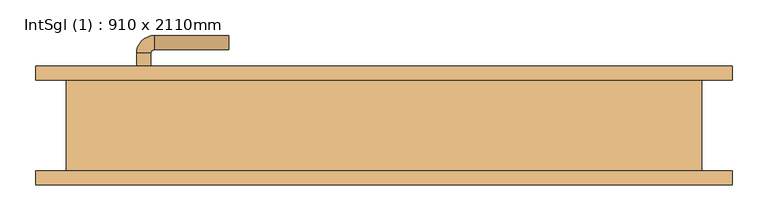
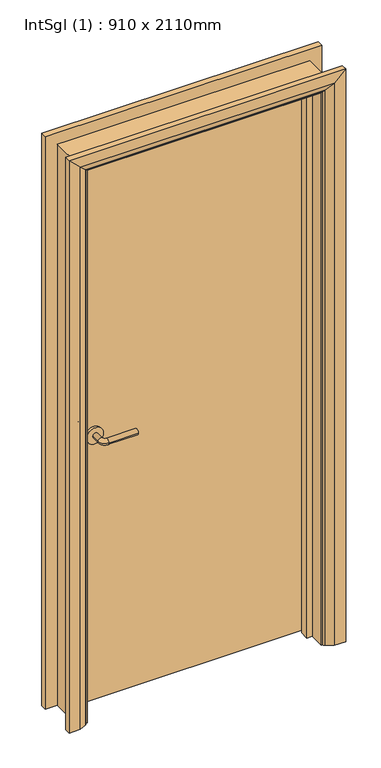
"""IFC4 building model written with IfcOpenShell, lengths in millimetres: door geometry, IntSgl (1) : 910 x 2110mm."""

import ifcopenshell
import ifcopenshell.guid

model = None  # the IFC model being written
_history = None  # IfcOwnerHistory: only IFC2X3 demands one
_inside = {}  # id of a spatial element -> (the spatial element, [elements in it])
_under = {}  # id of a project, library or spatial element -> (it, [spatial elements below it])
_declared = {}  # id of a project -> (the project, [libraries it declares])
_typed = {}  # id of a type object -> (the type object, [elements of that type])
_made_of = {}  # id of a material, layer set ... -> (it, [elements and type objects made of it])


def new_model(schema):
    """Start an empty IFC model of exactly this schema.

    Asked for "IFC4X3", IfcOpenShell would pick the latest addendum, in which some entities
    have other attributes; the version numbers below select the first issue.
    IFC2X3 requires an IfcOwnerHistory on every rooted entity: one is made here for all.
    """
    global model, _history
    if schema == "IFC4X3":
        model = ifcopenshell.file(schema_version=(4, 3, 0, 0))
    else:
        model = ifcopenshell.file(schema=schema)
    _inside.clear()
    _under.clear()
    _declared.clear()
    _typed.clear()
    _made_of.clear()
    _history = None
    if model.schema == "IFC2X3":
        org = make("IfcOrganization", Name="unknown")
        user = make(
            "IfcPersonAndOrganization",
            ThePerson=make("IfcPerson", FamilyName="unknown"),
            TheOrganization=org,
        )
        app = make(
            "IfcApplication",
            ApplicationDeveloper=org,
            Version="unknown",
            ApplicationFullName="unknown",
            ApplicationIdentifier="unknown",
        )
        _history = make(
            "IfcOwnerHistory",
            OwningUser=user,
            OwningApplication=app,
            ChangeAction="ADDED",
            CreationDate=0,
        )
    return model


def make(cls, **values):
    """One entity of the class cls with the attributes given. An attribute that is None is left unset."""
    return model.create_entity(
        cls, **{name: value for name, value in values.items() if value is not None}
    )


def rooted(cls, **values):
    """An entity with a GlobalId (a new one), such as an element, a storey or a relation."""
    return make(cls, GlobalId=ifcopenshell.guid.new(), OwnerHistory=_history, **values)


def si_unit(unit_type, name, prefix=None):
    """IfcSIUnit, for example si_unit("LENGTHUNIT", "METRE", prefix="MILLI")."""
    return make("IfcSIUnit", UnitType=unit_type, Prefix=prefix, Name=name)


def assignment(units):
    """IfcUnitAssignment: the units of a project."""
    return None if units is None else make("IfcUnitAssignment", Units=units)


def point(xyz):
    """IfcCartesianPoint."""
    return None if xyz is None else make("IfcCartesianPoint", Coordinates=xyz)


def direction(xyz):
    """IfcDirection."""
    return None if xyz is None else make("IfcDirection", DirectionRatios=xyz)


def frame(location, z_axis=None, x_axis=None):
    """IfcAxis2Placement3D, a coordinate frame: its origin and axes. An axis left out is left unset."""
    return make(
        "IfcAxis2Placement3D",
        Location=point(location),
        Axis=direction(z_axis),
        RefDirection=direction(x_axis),
    )


def frame_2d(location, x_axis=None):
    """IfcAxis2Placement2D, a coordinate frame in the plane: its origin and x axis."""
    return make(
        "IfcAxis2Placement2D", Location=point(location), RefDirection=direction(x_axis)
    )


def origin():
    """The frame at (0, 0, 0) with its axes left unset."""
    return frame((0.0, 0.0, 0.0))


def place(relative_to, where):
    """IfcLocalPlacement: puts the frame where relative to a parent placement (None: the world)."""
    return make(
        "IfcLocalPlacement", PlacementRelTo=relative_to, RelativePlacement=where
    )


def context(
    kind, dimensions, precision=None, world=None, true_north=None, identifier=None
):
    """IfcGeometricRepresentationContext, for example the 3D "Model" context."""
    return make(
        "IfcGeometricRepresentationContext",
        ContextIdentifier=identifier,
        ContextType=kind,
        CoordinateSpaceDimension=dimensions,
        Precision=precision,
        WorldCoordinateSystem=world,
        TrueNorth=true_north,
    )


def project(units=None, contexts=None):
    """IfcProject with its units and contexts."""
    return rooted(
        "IfcProject",
        Name="project",
        RepresentationContexts=contexts,
        UnitsInContext=assignment(units),
    )


def spatial(cls, under=None, at=None, **own):
    """A site, building, storey or space (cls), placed at a placement, below another one or the project."""
    s = rooted(cls, ObjectPlacement=at, **own)
    if under is not None:
        _under.setdefault(under.id(), (under, []))[1].append(s)
    return s


def polyline(points):
    """IfcPolyline through the points."""
    return make("IfcPolyline", Points=[point(p) for p in points])


def circle_curve(where, radius):
    """IfcCircle in the frame where."""
    return make("IfcCircle", Position=where, Radius=radius)


def ellipse_curve(where, semi_axis1, semi_axis2):
    """IfcEllipse in the frame where."""
    return make(
        "IfcEllipse", Position=where, SemiAxis1=semi_axis1, SemiAxis2=semi_axis2
    )


def trimmed(basis, trim1, trim2, sense, master):
    """IfcTrimmedCurve: the piece of a basis curve between two trims."""
    return make(
        "IfcTrimmedCurve",
        BasisCurve=basis,
        Trim1=trim1,
        Trim2=trim2,
        SenseAgreement=sense,
        MasterRepresentation=master,
    )


def segment(curve, same_sense, transition):
    """IfcCompositeCurveSegment."""
    return make(
        "IfcCompositeCurveSegment",
        Transition=transition,
        SameSense=same_sense,
        ParentCurve=curve,
    )


def composite_curve(segments, self_intersect=None):
    """IfcCompositeCurve: segments joined end to end."""
    return make("IfcCompositeCurve", Segments=segments, SelfIntersect=self_intersect)


def outline(outer, holes=None, kind="AREA"):
    """IfcArbitraryClosedProfileDef: a profile drawn as a closed curve; with holes, ...WithVoids."""
    if holes is None:
        return make("IfcArbitraryClosedProfileDef", ProfileType=kind, OuterCurve=outer)
    return make(
        "IfcArbitraryProfileDefWithVoids",
        ProfileType=kind,
        OuterCurve=outer,
        InnerCurves=holes,
    )


def extrude(swept, where, along, depth):
    """IfcExtrudedAreaSolid: the profile swept, set in the frame where, extruded along a direction by depth."""
    return make(
        "IfcExtrudedAreaSolid",
        SweptArea=swept,
        Position=where,
        ExtrudedDirection=direction(along),
        Depth=depth,
    )


def faces_of(points, faces, orient=None, outer=None):
    """IfcFace entities. A face is a list of loops; a loop is a list of indices into points, from 0.

    orient and outer hold one flag for each loop. By default every Orientation is true, the
    first loop of a face is its IfcFaceOuterBound and the others are IfcFaceBound.
    """
    made = []
    for i, loops in enumerate(faces):
        bounds = []
        for j, loop in enumerate(loops):
            is_outer = j == 0 if outer is None else outer[i][j]
            bounds.append(
                make(
                    "IfcFaceOuterBound" if is_outer else "IfcFaceBound",
                    Bound=make("IfcPolyLoop", Polygon=[points[k] for k in loop]),
                    Orientation=True if orient is None else orient[i][j],
                )
            )
        made.append(make("IfcFace", Bounds=bounds))
    return made


def faceted_brep(points, faces, orient=None, outer=None, voids=None):
    """IfcFacetedBrep: a solid bounded by flat faces; with voids (closed shells), ...WithVoids."""
    shared = [point(p) for p in points]
    hull = make("IfcClosedShell", CfsFaces=faces_of(shared, faces, orient, outer))
    if voids is None:
        return make("IfcFacetedBrep", Outer=hull)
    return make(
        "IfcFacetedBrepWithVoids",
        Outer=hull,
        Voids=[
            make(cls, CfsFaces=faces_of(shared, fs, o, b)) for cls, fs, o, b in voids
        ],
    )


def shape(context_of_items, identifier, shape_type, items):
    """IfcShapeRepresentation: the items that make up one representation, for example the "Body"."""
    return make(
        "IfcShapeRepresentation",
        ContextOfItems=context_of_items,
        RepresentationIdentifier=identifier,
        RepresentationType=shape_type,
        Items=items,
    )


def source(mapping_origin, context_of_items, identifier, shape_type, items):
    """IfcRepresentationMap: a shape defined once, which mapped items show again and again."""
    return make(
        "IfcRepresentationMap",
        MappingOrigin=mapping_origin,
        MappedRepresentation=shape(context_of_items, identifier, shape_type, items),
    )


def transform(
    local_origin,
    x_axis=None,
    y_axis=None,
    z_axis=None,
    scale=None,
    scale2=None,
    scale3=None,
    uniform=True,
):
    """IfcCartesianTransformationOperator3D, or its non-uniform kind. x_axis, y_axis, z_axis: its Axis1, 2, 3."""
    if uniform:
        return make(
            "IfcCartesianTransformationOperator3D",
            Axis1=direction(x_axis),
            Axis2=direction(y_axis),
            LocalOrigin=point(local_origin),
            Scale=scale,
            Axis3=direction(z_axis),
        )
    return make(
        "IfcCartesianTransformationOperator3DnonUniform",
        Axis1=direction(x_axis),
        Axis2=direction(y_axis),
        LocalOrigin=point(local_origin),
        Scale=scale,
        Axis3=direction(z_axis),
        Scale2=scale2,
        Scale3=scale3,
    )


def mapped(mapping_source, mapping_target):
    """IfcMappedItem: shows the shape of a source again, moved by a transform."""
    return make(
        "IfcMappedItem", MappingSource=mapping_source, MappingTarget=mapping_target
    )


def made_of(thing, what):
    """Note that an element or type object is made of a material, layer set ...; save() writes the relation."""
    if what is not None:
        _made_of.setdefault(what.id(), (what, []))[1].append(thing)
    return thing


def element(
    cls,
    number,
    at=None,
    inside=None,
    cuts=None,
    type_object=None,
    material=None,
    context=None,
    identifier="Body",
    shape_type=None,
    held_by="IfcProductDefinitionShape",
    body=None,
    shapes=None,
    **own,
):
    """One element of the class cls, such as IfcWall. Its Tag is "e" and its number.

    at: its placement. inside: the storey or other place that contains it. cuts: it is an
    opening in that element (IfcRelVoidsElement). A single representation is given by context,
    identifier, shape_type and body (its items); several are given by shapes. held_by: the class
    of the entity that holds the representations. save() writes the other relations.
    """
    e = rooted(cls, Tag="e%d" % number, ObjectPlacement=at, **own)
    if body is not None:
        shapes = [shape(context, identifier, shape_type, body)]
    if shapes is not None:
        e.Representation = make(held_by, Representations=shapes)
    if inside is not None:
        _inside.setdefault(inside.id(), (inside, []))[1].append(e)
    if cuts is not None:
        rooted(
            "IfcRelVoidsElement", RelatingBuildingElement=cuts, RelatedOpeningElement=e
        )
    if type_object is not None:
        _typed.setdefault(type_object.id(), (type_object, []))[1].append(e)
    return made_of(e, material)


def aggregate(whole, parts):
    """IfcRelAggregates: a whole, such as a stair, and the parts it consists of."""
    return rooted("IfcRelAggregates", RelatingObject=whole, RelatedObjects=parts)


def save(model, path):
    """Write the relations noted so far, then the file.

    IfcRelAggregates (storeys below a building ...), IfcRelContainedInSpatialStructure (elements
    in a storey), IfcRelDefinesByType, IfcRelAssociatesMaterial and IfcRelDeclares: one each for
    every whole, place, type object, material and project.
    """
    for whole, parts in _under.values():
        aggregate(whole, parts)
    for where, things in _inside.values():
        rooted(
            "IfcRelContainedInSpatialStructure",
            RelatedElements=things,
            RelatingStructure=where,
        )
    for kind, things in _typed.values():
        rooted("IfcRelDefinesByType", RelatedObjects=things, RelatingType=kind)
    for what, things in _made_of.values():
        rooted("IfcRelAssociatesMaterial", RelatedObjects=things, RelatingMaterial=what)
    for by, libraries in _declared.values():
        rooted("IfcRelDeclares", RelatingContext=by, RelatedDefinitions=libraries)
    model.write(path)


def plane_surface(at):
    """IfcPlane: the flat surface through the origin of the frame at, square to its z axis."""
    return make("IfcPlane", Position=at)


def cylinder_surface(at, radius):
    """IfcCylindricalSurface: all points at the distance radius from the z axis of the frame at."""
    return make("IfcCylindricalSurface", Position=at, Radius=radius)


def revolved_surface(curve, axis_point, axis_direction):
    """IfcSurfaceOfRevolution: the curve turned about the line through axis_point along axis_direction."""
    return make(
        "IfcSurfaceOfRevolution",
        SweptCurve=make("IfcArbitraryOpenProfileDef", ProfileType="CURVE", Curve=curve),
        AxisPosition=make("IfcAxis1Placement", Location=point(axis_point), Axis=direction(axis_direction)),
    )


def advanced_brep(points, edges, surfaces, faces):
    """IfcAdvancedBrep: a solid bounded by faces that lie on surfaces and meet in shared edges.

    An edge is (start, end): straight between two places in points (the first is 0);
    or (start, end, curve); or (start, end, curve, False) where it runs against its curve.
    A face is (place in surfaces, loops), or (place, loops, False) where it looks against
    its surface's normal. A loop lists edges by number (the first is 1), with a minus sign
    where the edge is run from its end to its start. The first loop is the outer one.
    """
    corners = [point(p) for p in points]
    vertices = [make("IfcVertexPoint", VertexGeometry=c) for c in corners]
    made = []
    for start, end, *more in edges:
        made.append(
            make(
                "IfcEdgeCurve",
                EdgeStart=vertices[start],
                EdgeEnd=vertices[end],
                EdgeGeometry=more[0] if more else make("IfcPolyline", Points=[corners[start], corners[end]]),
                SameSense=more[1] if len(more) > 1 else True,
            )
        )
    hull = []
    for where, loops, *sense in faces:
        bounds = []
        for j, loop in enumerate(loops):
            ring = [make("IfcOrientedEdge", EdgeElement=made[abs(k) - 1], Orientation=k > 0) for k in loop]
            bounds.append(
                make(
                    "IfcFaceOuterBound" if j == 0 else "IfcFaceBound",
                    Bound=make("IfcEdgeLoop", EdgeList=ring),
                    Orientation=True,
                )
            )
        hull.append(make("IfcAdvancedFace", Bounds=bounds, FaceSurface=surfaces[where], SameSense=sense[0] if sense else True))
    return make("IfcAdvancedBrep", Outer=make("IfcClosedShell", CfsFaces=hull))


def intsgl_1_910_x_2110mm_8bdb4243(model_context):
    return source(origin(), model_context, "Body", "SolidModel", [
        advanced_brep(
        [(-348.0, 17.75, 1000.0), (-328.0, 17.75, 1000.0), (-328.0, -12.25, 1000.0), (-348.0, -12.25, 1000.0), (-323.0, -17.25, 1000.0), (-323.0, -37.25, 1000.0), (-218.0, -37.25, 1000.0), (-218.0, -17.25, 1000.0)],
        [
            (0, 1, circle_curve(frame((-338.0, 17.75, 1000.0), z_axis=(0.0, 1.0, 0.0), x_axis=(1.0, 0.0, 0.0)), 10.0)),
            (1, 0, circle_curve(frame((-338.0, 17.75, 1000.0), z_axis=(0.0, 1.0, 0.0), x_axis=(1.0, 0.0, 0.0)), 10.0)),
            (1, 2),
            (2, 3, circle_curve(frame((-338.0, -12.25, 1000.0), z_axis=(0.0, 1.0, 0.0), x_axis=(1.0, 0.0, 0.0)), 10.0)),
            (3, 0),
            (3, 2, circle_curve(frame((-338.0, -12.25, 1000.0), z_axis=(0.0, 1.0, 0.0), x_axis=(1.0, 0.0, 0.0)), 10.0)),
            (4, 5, circle_curve(frame((-323.0, -27.25, 1000.0), z_axis=(-1.0, 0.0, 0.0), x_axis=(0.0, 1.0, 0.0)), 10.0)),
            (5, 3, circle_curve(frame((-323.0, -12.25, 1000.0), z_axis=(0.0, 0.0, -1.0), x_axis=(-1.0, 0.0, 0.0)), 25.0)),
            (2, 4, circle_curve(frame((-323.0, -12.25, 1000.0), z_axis=(0.0, 0.0, 1.0), x_axis=(-1.0, 0.0, 0.0)), 5.0)),
            (5, 4, circle_curve(frame((-323.0, -27.25, 1000.0), z_axis=(-1.0, 0.0, 0.0), x_axis=(0.0, 1.0, 0.0)), 10.0)),
            (6, 7, circle_curve(frame((-218.0, -27.25, 1000.0), z_axis=(1.0, 0.0, 0.0), x_axis=(0.0, 1.0, 0.0)), 10.0)),
            (7, 6, circle_curve(frame((-218.0, -27.25, 1000.0), z_axis=(1.0, 0.0, 0.0), x_axis=(0.0, 1.0, 0.0)), 10.0)),
            (4, 7),
            (6, 5),
        ],
        [
            plane_surface(frame((-338.0, 17.75, 1000.0), z_axis=(0.0, 1.0, 0.0), x_axis=(0.0, 0.0, 1.0))),
            cylinder_surface(frame((-338.0, 17.75, 1000.0), z_axis=(0.0, 1.0, 0.0), x_axis=(1.0, 0.0, 0.0)), 10.0),
            revolved_surface(trimmed(ellipse_curve(frame((-338.0, -12.25, 1000.0), z_axis=(0.0, -1.0, 0.0), x_axis=(1.0, 0.0, 0.0)), 10.0, 10.0), [point((-348.0, -12.25, 1000.0))], [point((-328.0, -12.25, 1000.0))], True, "CARTESIAN"), (-323.0, -12.25, 1000.0), (0.0, 0.0, -1.0)),
            revolved_surface(trimmed(ellipse_curve(frame((-338.0, -12.25, 1000.0), z_axis=(0.0, -1.0, 0.0), x_axis=(1.0, 0.0, 0.0)), 10.0, 10.0), [point((-328.0, -12.25, 1000.0))], [point((-348.0, -12.25, 1000.0))], True, "CARTESIAN"), (-323.0, -12.25, 1000.0), (0.0, 0.0, -1.0)),
            plane_surface(frame((-218.0, -27.25, 1000.0), z_axis=(1.0, 0.0, 0.0), x_axis=(0.0, 0.0, 1.0))),
            cylinder_surface(frame((-323.0, -27.25, 1000.0), z_axis=(-1.0, 0.0, 0.0), x_axis=(0.0, 1.0, 0.0)), 10.0),
        ],
        [
            (0, [[1, 2]]),
            (1, [[3, 4, 5, -2]]),
            (1, [[-5, 6, -3, -1]]),
            (2, [[7, 8, -4, 9]]),
            (3, [[10, -9, -6, -8]]),
            (4, [[11, 12]]),
            (5, [[13, -11, 14, -7]]),
            (5, [[-14, -12, -13, -10]]),
        ],
    ),
        extrude(outline(composite_curve([segment(trimmed(circle_curve(frame_2d((1000.0, -340.5)), 30.0), [point((1000.0, -370.5))], [point((1000.0, -310.5))], False, "CARTESIAN"), True, "CONTINUOUS"), segment(trimmed(circle_curve(frame_2d((1000.0, -340.5)), 30.0), [point((1000.0, -310.5))], [point((1000.0, -370.5))], False, "CARTESIAN"), True, "CONTINUOUS")], self_intersect=False)), frame((0.0, 17.75, 0.0), z_axis=(0.0, 1.0, 0.0), x_axis=(0.0, 0.0, 1.0)), (0.0, 0.0, 1.0), 8.0),
        advanced_brep(
        [(-348.0, 71.75, 1000.0), (-328.0, 71.75, 1000.0), (-348.0, 101.75, 1000.0), (-328.0, 101.75, 1000.0), (-323.0, 106.75, 1000.0), (-323.0, 126.75, 1000.0), (-218.0, 126.75, 1000.0), (-218.0, 106.75, 1000.0)],
        [
            (0, 1, circle_curve(frame((-338.0, 71.75, 1000.0), z_axis=(0.0, -1.0, 0.0), x_axis=(1.0, 0.0, 0.0)), 10.0)),
            (1, 0, circle_curve(frame((-338.0, 71.75, 1000.0), z_axis=(0.0, -1.0, 0.0), x_axis=(1.0, 0.0, 0.0)), 10.0)),
            (0, 2),
            (2, 3, circle_curve(frame((-338.0, 101.75, 1000.0), z_axis=(0.0, -1.0, 0.0), x_axis=(1.0, 0.0, 0.0)), 10.0)),
            (3, 1),
            (3, 2, circle_curve(frame((-338.0, 101.75, 1000.0), z_axis=(0.0, -1.0, 0.0), x_axis=(1.0, 0.0, 0.0)), 10.0)),
            (4, 3, circle_curve(frame((-323.0, 101.75, 1000.0), z_axis=(0.0, 0.0, 1.0), x_axis=(-1.0, 0.0, 0.0)), 5.0)),
            (2, 5, circle_curve(frame((-323.0, 101.75, 1000.0), z_axis=(0.0, 0.0, -1.0), x_axis=(-1.0, 0.0, 0.0)), 25.0)),
            (5, 4, circle_curve(frame((-323.0, 116.75, 1000.0), z_axis=(-1.0, 0.0, 0.0), x_axis=(0.0, -1.0, 0.0)), 10.0)),
            (4, 5, circle_curve(frame((-323.0, 116.75, 1000.0), z_axis=(-1.0, 0.0, 0.0), x_axis=(0.0, -1.0, 0.0)), 10.0)),
            (6, 7, circle_curve(frame((-218.0, 116.75, 1000.0), z_axis=(1.0, 0.0, 0.0), x_axis=(0.0, -1.0, 0.0)), 10.0)),
            (7, 6, circle_curve(frame((-218.0, 116.75, 1000.0), z_axis=(1.0, 0.0, 0.0), x_axis=(0.0, -1.0, 0.0)), 10.0)),
            (5, 6),
            (7, 4),
        ],
        [
            plane_surface(frame((-338.0, 71.75, 1000.0), z_axis=(0.0, -1.0, 0.0), x_axis=(0.0, 0.0, 1.0))),
            cylinder_surface(frame((-338.0, 71.75, 1000.0), z_axis=(0.0, -1.0, 0.0), x_axis=(1.0, 0.0, 0.0)), 10.0),
            revolved_surface(trimmed(ellipse_curve(frame((-338.0, 101.75, 1000.0), z_axis=(0.0, -1.0, 0.0), x_axis=(1.0, 0.0, 0.0)), 10.0, 10.0), [point((-348.0, 101.75, 1000.0))], [point((-328.0, 101.75, 1000.0))], True, "CARTESIAN"), (-323.0, 101.75, 1000.0), (0.0, 0.0, -1.0)),
            revolved_surface(trimmed(ellipse_curve(frame((-338.0, 101.75, 1000.0), z_axis=(0.0, -1.0, 0.0), x_axis=(1.0, 0.0, 0.0)), 10.0, 10.0), [point((-328.0, 101.75, 1000.0))], [point((-348.0, 101.75, 1000.0))], True, "CARTESIAN"), (-323.0, 101.75, 1000.0), (0.0, 0.0, -1.0)),
            plane_surface(frame((-218.0, 116.75, 1000.0), z_axis=(1.0, 0.0, 0.0), x_axis=(0.0, 0.0, 1.0))),
            cylinder_surface(frame((-323.0, 116.75, 1000.0), z_axis=(-1.0, 0.0, 0.0), x_axis=(0.0, -1.0, 0.0)), 10.0),
        ],
        [
            (0, [[1, 2]]),
            (1, [[-1, 3, 4, 5]]),
            (1, [[-2, -5, 6, -3]]),
            (2, [[7, -4, 8, 9]]),
            (3, [[-8, -6, -7, 10]]),
            (4, [[11, 12]]),
            (5, [[-9, 13, -12, 14]]),
            (5, [[-10, -14, -11, -13]]),
        ],
    ),
        extrude(outline(composite_curve([segment(trimmed(circle_curve(frame_2d((1000.0, -340.5)), 30.0), [point((1000.0, -370.5))], [point((1000.0, -310.5))], False, "CARTESIAN"), True, "CONTINUOUS"), segment(trimmed(circle_curve(frame_2d((1000.0, -340.5)), 30.0), [point((1000.0, -310.5))], [point((1000.0, -370.5))], False, "CARTESIAN"), True, "CONTINUOUS")], self_intersect=False)), frame((0.0, 63.75, 0.0), z_axis=(0.0, 1.0, 0.0), x_axis=(0.0, 0.0, 1.0)), (0.0, 0.0, 1.0), 8.0),
        extrude(outline(polyline([(413.0, 25.75), (-413.0, 25.75), (-413.0, 63.75), (413.0, 63.75), (413.0, 25.75)])), frame((0.0, 0.0, 8.0), z_axis=(0.0, 0.0, 1.0), x_axis=(1.0, 0.0, 0.0)), (0.0, 0.0, 1.0), 2060.0),
        advanced_brep(
        [(490.0, 83.75, 0.0), (490.0, 63.75, 0.0), (420.0, 63.75, 0.0), (424.0, 69.75, 0.0), (450.0, 83.75, 0.0), (490.0, 83.75, 2145.0), (490.0, 63.75, 2145.0), (-490.0, 63.75, 2145.0), (-490.0, 63.75, 0.0), (-420.0, 63.75, 0.0), (-420.0, 63.75, 2075.0), (420.0, 63.75, 2075.0), (424.0, 69.75, 2079.0), (450.0, 83.75, 2105.0), (-450.0, 83.75, 2105.0), (-450.0, 83.75, 0.0), (-490.0, 83.75, 0.0), (-490.0, 83.75, 2145.0), (-424.0, 69.75, 2079.0), (-424.0, 69.75, 0.0)],
        [
            (0, 1),
            (1, 2),
            (2, 3, circle_curve(frame((428.0, 62.75, 0.0), z_axis=(0.0, 0.0, -1.0), x_axis=(1.0, 0.0, 0.0)), 8.0622577)),
            (3, 4),
            (4, 0),
            (0, 5),
            (5, 6),
            (6, 1),
            (6, 7),
            (7, 8),
            (8, 9),
            (9, 10),
            (10, 11),
            (11, 2),
            (11, 12, ellipse_curve(frame((428.0, 62.75, 2083.0), z_axis=(0.7071067811865475, 0.0, -0.7071067811865475), x_axis=(-0.7071067811865474, 0.0, -0.7071067811865476)), 11.4017543, 8.0622577)),
            (12, 3),
            (12, 13),
            (13, 4),
            (13, 14),
            (14, 15),
            (15, 16),
            (16, 17),
            (17, 5),
            (17, 7),
            (10, 18, ellipse_curve(frame((-428.0, 62.75, 2083.0), z_axis=(0.7071067811865475, 0.0, 0.7071067811865475), x_axis=(0.7071067811865476, 0.0, -0.7071067811865474)), 11.4017543, 8.0622577)),
            (18, 12),
            (18, 14),
            (15, 19),
            (19, 9, circle_curve(frame((-428.0, 62.75, 0.0), z_axis=(0.0, 0.0, -1.0), x_axis=(-1.0, 0.0, 0.0)), 8.0622577)),
            (8, 16),
            (19, 18),
        ],
        [
            plane_surface(frame((420.0, 63.75, 0.0), z_axis=(0.0, 0.0, -1.0), x_axis=(0.0, -1.0, 0.0))),
            plane_surface(frame((490.0, 83.75, 0.0), z_axis=(1.0, 0.0, 0.0), x_axis=(0.0, 0.0, 1.0))),
            plane_surface(frame((490.0, 63.75, 0.0), z_axis=(0.0, -1.0, 0.0), x_axis=(0.0, 0.0, 1.0))),
            cylinder_surface(frame((428.0, 62.75, 0.0), z_axis=(0.0, 0.0, -1.0), x_axis=(1.0, 0.0, 0.0)), 8.0622577),
            plane_surface(frame((424.0, 69.75, 0.0), z_axis=(-0.4740998230350126, 0.880471099922178, 0.0), x_axis=(0.0, 0.0, 1.0))),
            plane_surface(frame((450.0, 83.75, 0.0), z_axis=(0.0, 1.0, 0.0), x_axis=(0.0, 0.0, 1.0))),
            plane_surface(frame((490.0, 83.75, 2145.0), z_axis=(0.0, 0.0, 1.0), x_axis=(-1.0, 0.0, 0.0))),
            cylinder_surface(frame((420.0, 62.75, 2083.0), z_axis=(1.0, 0.0, 0.0), x_axis=(0.0, 0.0, 1.0)), 8.0622577),
            plane_surface(frame((424.0, 69.75, 2079.0), z_axis=(0.0, 0.8804710999221764, -0.4740998230350154), x_axis=(-1.0, 0.0, 0.0))),
            plane_surface(frame((-420.0, 63.75, 0.0), z_axis=(0.0, 0.0, -1.0), x_axis=(0.0, -1.0, 0.0))),
            plane_surface(frame((-490.0, 83.75, 2145.0), z_axis=(-1.0, 0.0, 0.0), x_axis=(0.0, 0.0, -1.0))),
            cylinder_surface(frame((-428.0, 62.75, 2075.0), z_axis=(0.0, 0.0, 1.0), x_axis=(-1.0, 0.0, 0.0)), 8.0622577),
            plane_surface(frame((-424.0, 69.75, 2079.0), z_axis=(0.47409982303501824, 0.8804710999221749, 0.0), x_axis=(0.0, 0.0, -1.0))),
        ],
        [
            (0, [[1, 2, 3, 4, 5]]),
            (1, [[-1, 6, 7, 8]]),
            (2, [[-2, -8, 9, 10, 11, 12, 13, 14]]),
            (3, [[-3, -14, 15, 16]]),
            (4, [[-4, -16, 17, 18]]),
            (5, [[-5, -18, 19, 20, 21, 22, 23, -6]]),
            (6, [[-7, -23, 24, -9]]),
            (7, [[-15, -13, 25, 26]]),
            (8, [[-17, -26, 27, -19]]),
            (9, [[-21, 28, 29, -11, 30]]),
            (10, [[-24, -22, -30, -10]]),
            (11, [[-25, -12, -29, 31]]),
            (12, [[-27, -31, -28, -20]]),
        ],
    ),
        extrude(outline(polyline([(0.0, -415.0), (0.0, -396.0), (2051.0, -396.0), (2051.0, 396.0), (0.0, 396.0), (0.0, 415.0), (2070.0, 415.0), (2070.0, -415.0), (0.0, -415.0)])), frame((0.0, -8.25, 0.0), z_axis=(0.0, 1.0, 0.0), x_axis=(0.0, 0.0, 1.0)), (0.0, 0.0, 1.0), 32.0),
        advanced_brep(
        [(-490.0, -83.75, 0.0), (-490.0, -63.75, 0.0), (-420.0, -63.75, 0.0), (-424.0, -69.75, 0.0), (-450.0, -83.75, 0.0), (-490.0, -83.75, 2145.0), (-490.0, -63.75, 2145.0), (-420.0, -63.75, 2075.0), (-424.0, -69.75, 2079.0), (-450.0, -83.75, 2105.0), (490.0, -83.75, 2145.0), (490.0, -63.75, 2145.0), (420.0, -63.75, 2075.0), (424.0, -69.75, 2079.0), (450.0, -83.75, 2105.0), (490.0, -83.75, 0.0), (450.0, -83.75, 0.0), (424.0, -69.75, 0.0), (420.0, -63.75, 0.0), (490.0, -63.75, 0.0)],
        [
            (0, 1),
            (1, 2),
            (2, 3, circle_curve(frame((-428.0, -62.75, 0.0), z_axis=(0.0, 0.0, -1.0), x_axis=(-1.0, 0.0, 0.0)), 8.0622577)),
            (3, 4),
            (4, 0),
            (0, 5),
            (5, 6),
            (6, 1),
            (6, 7),
            (7, 2),
            (7, 8, ellipse_curve(frame((-428.0, -62.75, 2083.0), z_axis=(-0.7071067811865475, 0.0, -0.7071067811865475), x_axis=(0.7071067811865474, 0.0, -0.7071067811865476)), 11.4017543, 8.0622577)),
            (8, 3),
            (8, 9),
            (9, 4),
            (9, 5),
            (5, 10),
            (10, 11),
            (11, 6),
            (11, 12),
            (12, 7),
            (12, 13, ellipse_curve(frame((428.0, -62.75, 2083.0), z_axis=(-0.7071067811865475, 0.0, 0.7071067811865475), x_axis=(-0.7071067811865476, 0.0, -0.7071067811865474)), 11.4017543, 8.0622577)),
            (13, 8),
            (13, 14),
            (14, 9),
            (14, 10),
            (15, 16),
            (16, 17),
            (17, 18, circle_curve(frame((428.0, -62.75, 0.0), z_axis=(0.0, 0.0, -1.0), x_axis=(1.0, 0.0, 0.0)), 8.0622577)),
            (18, 19),
            (19, 15),
            (10, 15),
            (19, 11),
            (18, 12),
            (17, 13),
            (16, 14),
        ],
        [
            plane_surface(frame((-420.0, -136.5510989, 0.0), z_axis=(0.0, 0.0, -1.0), x_axis=(1.0, 0.0, 0.0))),
            plane_surface(frame((-490.0, -83.75, 0.0), z_axis=(-1.0, 0.0, 0.0), x_axis=(0.0, 0.0, 1.0))),
            plane_surface(frame((-490.0, -63.75, 0.0), z_axis=(0.0, 1.0, 0.0), x_axis=(0.0, 0.0, 1.0))),
            cylinder_surface(frame((-428.0, -62.75, 0.0), z_axis=(0.0, 0.0, -1.0), x_axis=(-1.0, 0.0, 0.0)), 8.0622577),
            plane_surface(frame((-424.0, -69.75, 0.0), z_axis=(0.4740998230350183, -0.8804710999221749, 0.0), x_axis=(0.0, 0.0, 1.0))),
            plane_surface(frame((-450.0, -83.75, 0.0), z_axis=(0.0, -1.0, 0.0), x_axis=(0.0, 0.0, 1.0))),
            plane_surface(frame((-490.0, -83.75, 2145.0), z_axis=(0.0, 0.0, 1.0), x_axis=(1.0, 0.0, 0.0))),
            plane_surface(frame((-490.0, -63.75, 2145.0), z_axis=(0.0, 1.0, 0.0), x_axis=(1.0, 0.0, 0.0))),
            cylinder_surface(frame((-420.0, -62.75, 2083.0), z_axis=(-1.0, 0.0, 0.0), x_axis=(0.0, 0.0, 1.0)), 8.0622577),
            plane_surface(frame((-424.0, -69.75, 2079.0), z_axis=(0.0, -0.8804710999221749, -0.4740998230350183), x_axis=(1.0, 0.0, 0.0))),
            plane_surface(frame((-450.0, -83.75, 2105.0), z_axis=(0.0, -1.0, 0.0), x_axis=(1.0, 0.0, 0.0))),
            plane_surface(frame((420.0, -136.5510989, 0.0), z_axis=(0.0, 0.0, -1.0), x_axis=(-1.0, 0.0, 0.0))),
            plane_surface(frame((490.0, -83.75, 2145.0), z_axis=(1.0, 0.0, 0.0), x_axis=(0.0, 0.0, -1.0))),
            plane_surface(frame((490.0, -63.75, 2145.0), z_axis=(0.0, 1.0, 0.0), x_axis=(0.0, 0.0, -1.0))),
            cylinder_surface(frame((428.0, -62.75, 2075.0), z_axis=(0.0, 0.0, 1.0), x_axis=(1.0, 0.0, 0.0)), 8.0622577),
            plane_surface(frame((424.0, -69.75, 2079.0), z_axis=(-0.4740998230350183, -0.8804710999221749, 0.0), x_axis=(0.0, 0.0, -1.0))),
            plane_surface(frame((450.0, -83.75, 2105.0), z_axis=(0.0, -1.0, 0.0), x_axis=(0.0, 0.0, -1.0))),
        ],
        [
            (0, [[1, 2, 3, 4, 5]]),
            (1, [[-1, 6, 7, 8]]),
            (2, [[-2, -8, 9, 10]]),
            (3, [[-3, -10, 11, 12]]),
            (4, [[-4, -12, 13, 14]]),
            (5, [[-5, -14, 15, -6]]),
            (6, [[-7, 16, 17, 18]]),
            (7, [[-9, -18, 19, 20]]),
            (8, [[-11, -20, 21, 22]]),
            (9, [[-13, -22, 23, 24]]),
            (10, [[-15, -24, 25, -16]]),
            (11, [[26, 27, 28, 29, 30]]),
            (12, [[-17, 31, -30, 32]]),
            (13, [[-19, -32, -29, 33]]),
            (14, [[-21, -33, -28, 34]]),
            (15, [[-23, -34, -27, 35]]),
            (16, [[-25, -35, -26, -31]]),
        ],
    ),
        faceted_brep([(-415.0, 63.75, 0.0), (-415.0, -63.75, 0.0), (-447.0, -63.75, 0.0), (-447.0, 63.75, 0.0), (-415.0, 63.75, 2070.0), (-415.0, -63.75, 2070.0), (-447.0, -63.75, 2102.0), (-447.0, 63.75, 2102.0), (415.0, 63.75, 2070.0), (415.0, -63.75, 2070.0), (447.0, -63.75, 2102.0), (447.0, 63.75, 2102.0), (415.0, 63.75, 0.0), (447.0, 63.75, 0.0), (447.0, -63.75, 0.0), (415.0, -63.75, 0.0)], [[[0, 1, 2, 3]], [[1, 0, 4, 5]], [[2, 1, 5, 6]], [[3, 2, 6, 7]], [[0, 3, 7, 4]], [[5, 4, 8, 9]], [[6, 5, 9, 10]], [[7, 6, 10, 11]], [[4, 7, 11, 8]], [[12, 13, 14, 15]], [[9, 8, 12, 15]], [[10, 9, 15, 14]], [[11, 10, 14, 13]], [[8, 11, 13, 12]]]),
    ])


if __name__ == "__main__":
    model = new_model("IFC4")
    model_context = context("Model", 3, world=origin())
    ifc_project = project(units=[si_unit("LENGTHUNIT", "METRE", prefix="MILLI")], contexts=[model_context])
    site = spatial("IfcSite", under=ifc_project)
    building = spatial("IfcBuilding", under=site)
    placement = place(None, origin())
    intsgl_1_910_x_2110mm_shape = intsgl_1_910_x_2110mm_8bdb4243(model_context)
    element("IfcDoor", 1, ObjectType="IntSgl (1) : 910 x 2110mm", at=placement, inside=building, context=model_context, shape_type="MappedRepresentation", body=[
        mapped(intsgl_1_910_x_2110mm_shape, transform((0.0, 0.0, 0.0), x_axis=(1.0, 0.0, 0.0), y_axis=(0.0, 1.0, 0.0), z_axis=(0.0, 0.0, 1.0))),
    ])
    save(model, "model.ifc")

# Revit data of these elements
# Type "IntSgl (1) : 910 x 2110mm"
#   Construction Type Id = "MDOOR"
#   Analytic Construction = "Metal"
#   Type Mark = "41"
#   Type Comments = "Internal Single"
#   Operation = "SingleSwingRight"
#   Manufacturer = "Revit"
#   Keynote = "L20"
#   Description = "Internal Single Door"
#   Visual Light Transmittance = 0
#   Solar Heat Gain Coefficient = 0
#   Heat Transfer Coefficient (U) = 3.7021 W/(m²·K)
#   UnderCut = 8 mm
#   Tolerance = 2 mm
#   Thickness = 38 mm
#   Structural Tolerance = 8 mm
#   StopDepth = 32 mm
#   Stop Thickness = 19 mm
#   Rough Width = 910 mm
#   Rough Height = 2110 mm
#   Height to Top Lock Rail = 1000 mm
#   Handle Z Distance = 1000 mm
#   Handle X Distance = 75 mm
#   Frame Thickness = 32 mm
#   Door Panel Width = 826 mm
#   Door Panel Thickness = 38 mm
#   Door Panel Offset = 0 mm
#   Height = 2110 mm
#   Width = 910 mm
#   Door Panel Height = 2060 mm
#   Architrave Setback = 5 mm
#   Function = 0
#   Vis - Ironmongery = yes
#   Material Ironmongery = Door - Handle
#   Material Frame = Door - Frame/Mullion (1)
#   Material Door = Door - Panel
#   Material Architrave = Door - Architrave
#   Wall Closure = (empty or 0)
# Element 1 (IfcDoor, "IntSgl (1) : 910 x 2110mm")
#   Materials on its faces: "Door - Architrave", "Door - Handle", "Door - Frame/Mullion (1)", "Door - Panel"
# Materials
#   "Door - Handle": class "Miscellaneous", colour RGB 0 0 0, transparency 0, Keynote = "P21"
#   "Door - Frame/Mullion (1)": class "Wood", colour RGB 212 179 113, transparency 0, Keynote = "L20", Cost = 0
#   "Door - Panel": class "Wood", colour RGB 210 159 95, transparency 0, Keynote = "L20"
#   "Door - Architrave": class "Wood", colour RGB 154 90 5, transparency 0, Keynote = "P20"
